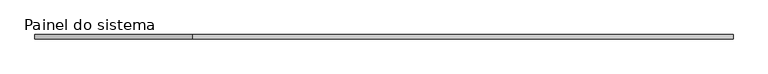
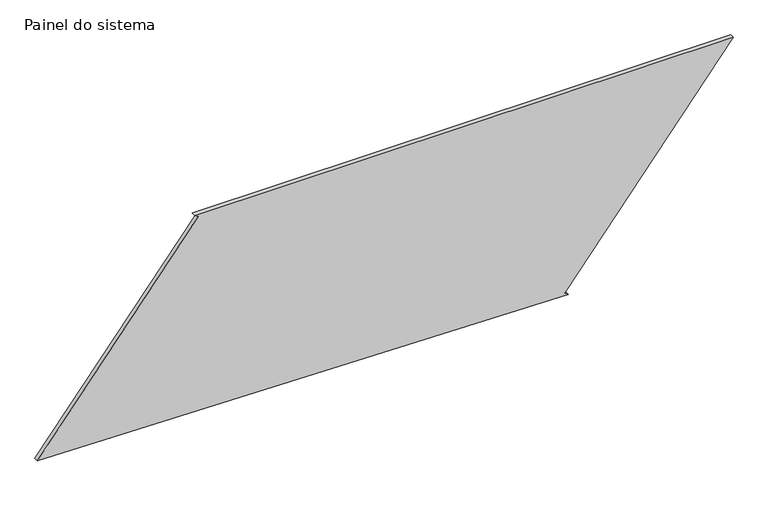
"""IFC4 building model written with IfcOpenShell, lengths in millimetres: plate geometry, Painel do sistema : Envidraçado."""

from ifc_helpers import new_model, si_unit, frame, origin, place, context, project, spatial, polyline, outline, extrude, source, transform, mapped, element, save


def painel_do_sistema_69a67380(model_context):
    return source(origin(), model_context, "Body", "SweptSolid", [
        extrude(outline(polyline([(0.0, 1105.502364), (15.5601026, 1085.9349624), (1295.3369982, 2103.6204068), (1295.3369982, -1151.3198586), (1279.7768956, -1131.752457), (57.6171855, -2103.6204068), (0.0, 1105.502364)])), frame((0.0, 24.5, 0.0), z_axis=(0.0, 1.0, 0.0), x_axis=(0.0, 0.0, 1.0)), (0.0, 0.0, 1.0), 25.0),
    ])


if __name__ == "__main__":
    model = new_model("IFC4")
    model_context = context("Model", 3, world=origin())
    ifc_project = project(units=[si_unit("LENGTHUNIT", "METRE", prefix="MILLI")], contexts=[model_context])
    site = spatial("IfcSite", under=ifc_project)
    building = spatial("IfcBuilding", under=site)
    placement = place(None, origin())
    painel_do_sistema_shape = painel_do_sistema_69a67380(model_context)
    element("IfcPlate", 1, ObjectType="Painel do sistema : Envidraçado", at=placement, inside=building, context=model_context, shape_type="MappedRepresentation", body=[
        mapped(painel_do_sistema_shape, transform((0.0, 0.0, 0.0), x_axis=(1.0, 0.0, 0.0), y_axis=(0.0, 1.0, 0.0), z_axis=(0.0, 0.0, 1.0))),
    ])
    save(model, "model.ifc")

# Revit data of these elements
# Type "Painel do sistema : Envidraçado"
#   Construction Type Id = "GSP4R"
#   Analytic Construction = "Vidraça única Pilkington 1/8 pol"
#   Visual Light Transmittance = 0.9
#   Solar Heat Gain Coefficient = 0.86
#   Heat Transfer Coefficient (U) = 6.7069 W/(m²·K)
# Element 1 (IfcPlate, "Painel do sistema : Envidraçado")
#   Materials on its faces: "Vidro"
# Materials
#   "Vidro": class "Vidro", colour RGB 0 128 192, transparency 0.9, Description = "Vidro de sílica", Cost = 0
